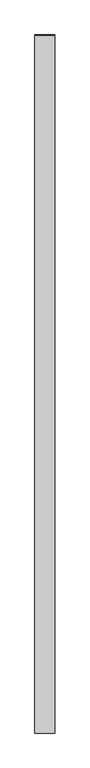
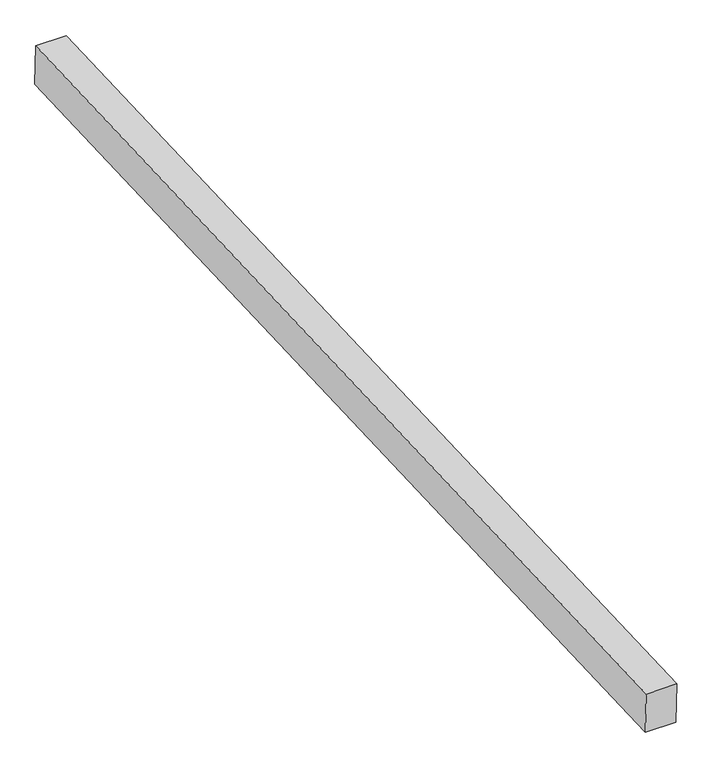
"""IFC4 building model written with IfcOpenShell, lengths in millimetres: proxy geometry, Generic Models 7:Generic Models 1:8:Generic Models 1:8 : Generic Models 7:Generic Models 1:337419:28 : Generic Models 7:Generic Models 1:8:Generic Models 1:8 : Generic Models 7:Generic Models 1:337419:315935."""

from ifc_helpers import new_model, si_unit, frame, origin, place, context, project, spatial, polyline, outline, extrude, source, transform, mapped, element, save


def generic_models_b2ba91c5(model_context):
    return source(origin(), model_context, "Body", "SweptSolid", [
        extrude(outline(polyline([(-569809.5331551, 8697.9424054), (-564936.6102609, 8900.9808594), (-564929.0433392, 8710.6308549), (-569801.6025364, 8507.607555), (-569809.5331551, 8697.9424054)])), frame((589988.4117243, 0.0, 0.0), z_axis=(1.0, 0.0, 0.0), x_axis=(0.0, 1.0, 0.0)), (0.0, 0.0, 1.0), 139.7),
    ])


if __name__ == "__main__":
    model = new_model("IFC4")
    model_context = context("Model", 3, world=origin())
    ifc_project = project(units=[si_unit("LENGTHUNIT", "METRE", prefix="MILLI")], contexts=[model_context])
    site = spatial("IfcSite", under=ifc_project)
    building = spatial("IfcBuilding", under=site)
    placement = place(None, origin())
    generic_models_shape = generic_models_b2ba91c5(model_context)
    element("IfcBuildingElementProxy", 1, Name="Generic Models 7:Generic Models 1:8:Generic Models 1:8 : Generic Models 7:Generic Models 1:337419:28 : Generic Models 7:Generic Models 1:8:Generic Models 1:8 : Generic Models 7:Generic Models 1:337419:315935", ObjectType="Generic Models 7:Generic Models 1:8:Generic Models 1:8 : Generic Models 7:Generic Models 1:337419:28 : Generic Models 7:Generic Models 1:8:Generic Models 1:8 : Generic Models 7:Generic Models 1:337419:315935", at=placement, inside=building, context=model_context, shape_type="MappedRepresentation", body=[
        mapped(generic_models_shape, transform((0.0, 0.0, 0.0), x_axis=(1.0, 0.0, 0.0), y_axis=(0.0, 1.0, 0.0), z_axis=(0.0, 0.0, 1.0))),
    ])
    save(model, "model.ifc")

# Revit data of these elements
# Type "Generic Models 7:Generic Models 1:8:Generic Models 1:8 : Generic Models 7:Generic Models 1:337419:28 : Generic Models 7:Generic Models 1:8:Generic Models 1:8 : Generic Models 7:Generic Models 1:337419:315935"
#   NameOverride = "Generic Models 7:Generic Models 1:8:Generic Models 1:8 : Generic Models 7:Generic Models 1:337419:315935"
#   ObjectTypeOverride = "Generic Models 1:8 : Generic Models 7:Generic Models 1:337419"
#   Reference = "Generic Models 1"
#   Tag = "315935"
# Element 1 (IfcBuildingElementProxy, "Generic Models 7:Generic Models 1:8:Generic Models 1:8 : Generic Models 7:Generic Models 1:337419:28 : Generic Models 7:Generic Models 1:8:Generic Models 1:8 : Generic Models 7:Generic Models 1:337419:315935")
#   Materials on its faces: "5 1/2\" X 7 1/2\" EXTERIOR GRADE GLULAM BEAMS"
# Materials
#   "5 1/2\" X 7 1/2\" EXTERIOR GRADE GLULAM BEAMS": class "Wood", colour RGB 183 134 68, transparency 0, Keynote = "M06181300.01", Description = "Pinus Echinata", Cost = 0
